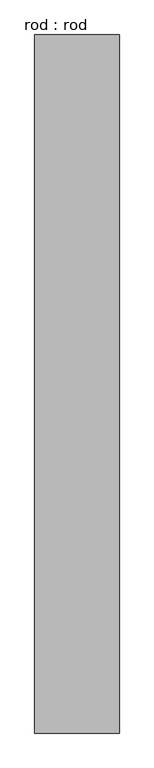
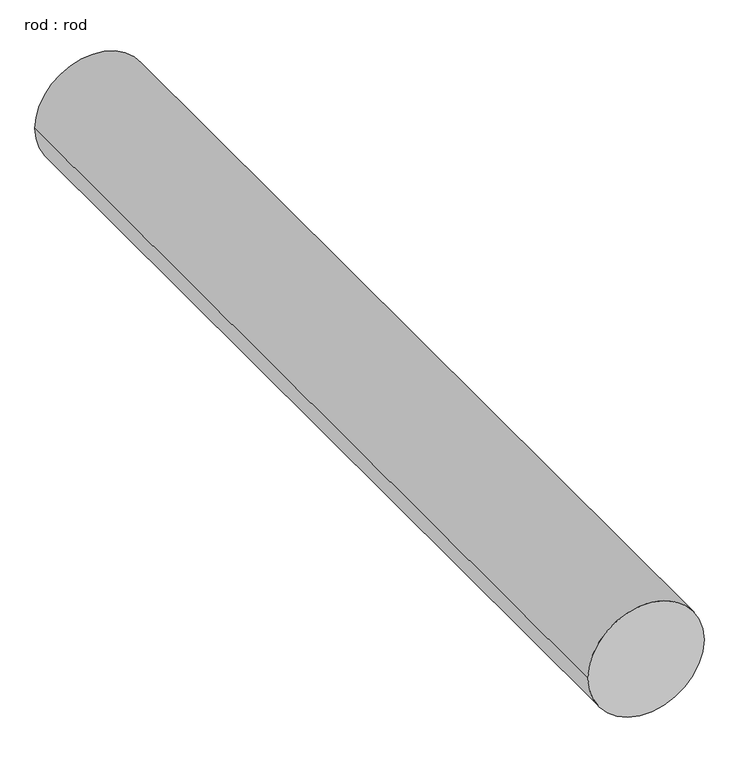
"""IFC4 building model written with IfcOpenShell, lengths in millimetres: proxy geometry, rod : rod."""

from ifc_helpers import new_model, si_unit, point, frame, frame_2d, origin, place, context, project, spatial, circle_curve, trimmed, segment, composite_curve, outline, extrude, source, transform, mapped, element, save


def rod_rod_6886257f(model_context):
    return source(origin(), model_context, "Body", "SweptSolid", [
        extrude(outline(composite_curve([segment(trimmed(circle_curve(frame_2d((0.0108462, 0.0)), 200.0), [point((0.0108462, 200.0))], [point((0.0108462, -200.0))], False, "CARTESIAN"), True, "CONTINUOUS"), segment(trimmed(circle_curve(frame_2d((0.0108462, 0.0)), 200.0), [point((0.0108462, -200.0))], [point((0.0108462, 200.0))], False, "CARTESIAN"), True, "CONTINUOUS")], self_intersect=False)), frame((0.0, 2442.7286153, 0.0), z_axis=(0.0, 1.0, 0.0), x_axis=(0.0, 0.0, 1.0)), (0.0, 0.0, 1.0), 3300.0),
    ])


if __name__ == "__main__":
    model = new_model("IFC4")
    model_context = context("Model", 3, world=origin())
    ifc_project = project(units=[si_unit("LENGTHUNIT", "METRE", prefix="MILLI")], contexts=[model_context])
    site = spatial("IfcSite", under=ifc_project)
    building = spatial("IfcBuilding", under=site)
    placement = place(None, origin())
    rod_rod_shape = rod_rod_6886257f(model_context)
    element("IfcBuildingElementProxy", 1, Name="rod : rod", ObjectType="rod : rod", at=placement, inside=building, context=model_context, shape_type="MappedRepresentation", body=[
        mapped(rod_rod_shape, transform((0.0, 0.0, 0.0), x_axis=(1.0, 0.0, 0.0), y_axis=(0.0, 1.0, 0.0), z_axis=(0.0, 0.0, 1.0))),
    ])
    save(model, "model.ifc")

# Revit data of these elements
# Type "rod : rod"
#   Default Elevation = 0
